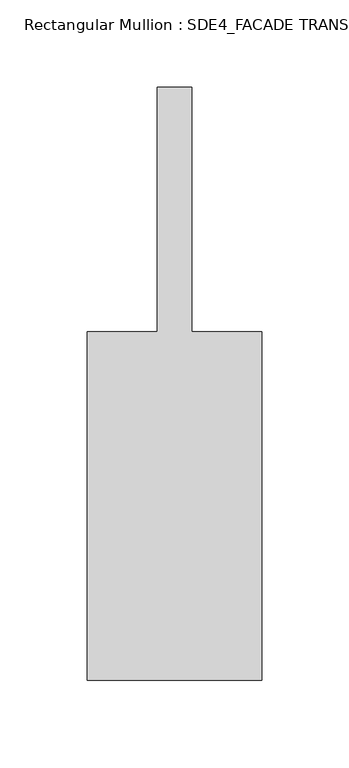
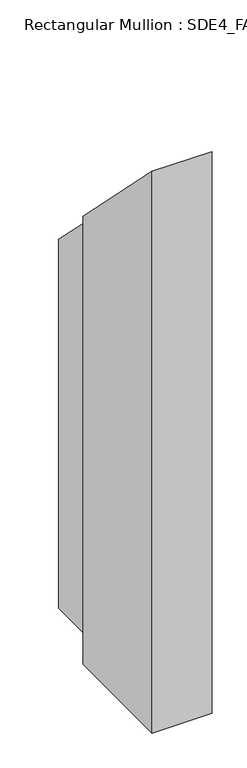
"""IFC4 building model written with IfcOpenShell, lengths in millimetres: member geometry, Rectangular Mullion : SDE4_FACADE TRANSOM TYPE 1."""

from ifc_helpers import new_model, si_unit, origin, place, context, project, spatial, faceted_brep, source, transform, mapped, element, save


def rectangular_mullion_sde4_facade_transom_type_1_77d7f65b(model_context):
    return source(origin(), model_context, "Body", "Brep", [
        faceted_brep([(50.0, -132.5, -859.5375289), (-50.0, -132.5, -859.5375289), (-50.0, 67.5, -859.5375289), (-10.0, 67.5, -859.5375289), (-10.0, 207.5, -859.5375289), (10.0, 207.5, -859.5375289), (10.0, 67.5, -859.5375289), (50.0, 67.5, -859.5375289), (50.0, 67.5, -67.5), (50.0, -132.5, 132.5), (10.0, 67.5, -67.5), (10.0, 207.5, -207.5), (-10.0, 207.5, -207.5), (-10.0, 67.5, -67.5), (-50.0, 67.5, -67.5), (-50.0, -132.5, 132.5)], [[[0, 1, 2, 3, 4, 5, 6, 7]], [[8, 9, 0, 7]], [[10, 8, 7, 6]], [[11, 10, 6, 5]], [[12, 11, 5, 4]], [[13, 12, 4, 3]], [[14, 13, 3, 2]], [[15, 14, 2, 1]], [[9, 15, 1, 0]], [[9, 8, 10, 11, 12, 13, 14, 15]]]),
    ])


if __name__ == "__main__":
    model = new_model("IFC4")
    model_context = context("Model", 3, world=origin())
    ifc_project = project(units=[si_unit("LENGTHUNIT", "METRE", prefix="MILLI")], contexts=[model_context])
    site = spatial("IfcSite", under=ifc_project)
    building = spatial("IfcBuilding", under=site)
    placement = place(None, origin())
    rectangular_mullion_sde4_facade_transom_type_1_shape = rectangular_mullion_sde4_facade_transom_type_1_77d7f65b(model_context)
    element("IfcMember", 1, ObjectType="Rectangular Mullion : SDE4_FACADE TRANSOM TYPE 1", at=placement, inside=building, context=model_context, shape_type="MappedRepresentation", body=[
        mapped(rectangular_mullion_sde4_facade_transom_type_1_shape, transform((0.0, 0.0, 0.0), x_axis=(1.0, 0.0, 0.0), y_axis=(0.0, 1.0, 0.0), z_axis=(0.0, 0.0, 1.0))),
    ])
    save(model, "model.ifc")

# Revit data of these elements
# Type "Rectangular Mullion : SDE4_FACADE TRANSOM TYPE 1"
#   built-in parameter 1007322 = 1.11549 (stored number, unit not read)
#   built-in parameter 1007321 = 0.164042 (stored number, unit not read)
#   built-in parameter 1007320 = 0.164042 (stored number, unit not read)
